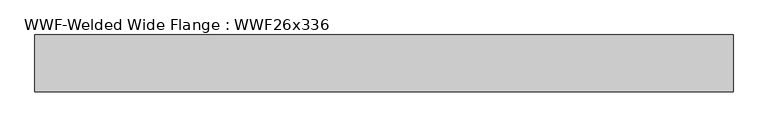
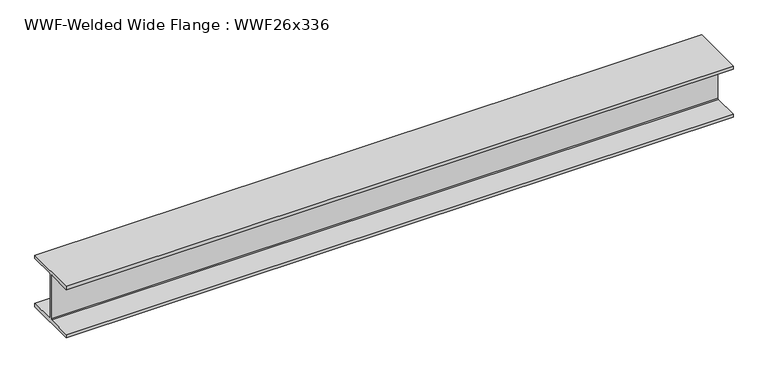
"""IFC4 building model written with IfcOpenShell, lengths in millimetres: beam geometry, WWF-Welded Wide Flange : WWF26x336."""

from ifc_helpers import new_model, si_unit, frame, origin, place, context, project, spatial, polyline, outline, extrude, source, transform, mapped, element, save


def wwf_welded_wide_flange_wwf26x336_095dbc8f(model_context):
    return source(origin(), model_context, "Body", "SweptSolid", [
        extrude(outline(polyline([(324.993, -284.988), (324.993, -324.993), (-324.993, -324.993), (-324.993, -284.988), (-20.6375, -284.988), (-9.9949, -274.3454), (-9.9949, 274.3454), (-20.6375, 284.988), (-324.993, 284.988), (-324.993, 324.993), (324.993, 324.993), (324.993, 284.988), (20.6375, 284.988), (9.9949, 274.3454), (9.9949, -274.3454), (20.6375, -284.988), (324.993, -284.988)])), frame((-3827.7582557, 0.0, 0.0), z_axis=(1.0, 0.0, 0.0), x_axis=(0.0, 1.0, 0.0)), (0.0, 0.0, 1.0), 7985.2423332),
    ])


if __name__ == "__main__":
    model = new_model("IFC4")
    model_context = context("Model", 3, world=origin())
    ifc_project = project(units=[si_unit("LENGTHUNIT", "METRE", prefix="MILLI")], contexts=[model_context])
    site = spatial("IfcSite", under=ifc_project)
    building = spatial("IfcBuilding", under=site)
    placement = place(None, origin())
    wwf_welded_wide_flange_wwf26x336_shape = wwf_welded_wide_flange_wwf26x336_095dbc8f(model_context)
    element("IfcBeam", 1, ObjectType="WWF-Welded Wide Flange : WWF26x336", at=placement, inside=building, context=model_context, shape_type="MappedRepresentation", body=[
        mapped(wwf_welded_wide_flange_wwf26x336_shape, transform((0.0, 0.0, 0.0), x_axis=(1.0, 0.0, 0.0), y_axis=(0.0, 1.0, 0.0), z_axis=(0.0, 0.0, 1.0))),
    ])
    save(model, "model.ifc")

# Revit data of these elements
# Type "WWF-Welded Wide Flange : WWF26x336"
#   Assembly Code = "B10"
#   Nominal d = "12"
#   W = 336
#   Length [instance default] = 1524 mm
#   bf = 649.986 mm
#   d = 649.986 mm
#   k = 20.638 mm
#   tf = 40.005 mm
#   tw = 19.99 mm
#   A = 0.0635483 m²
#   Structural Material [instance default] = Steel ASTM A572
# Element 1 (IfcBeam, "WWF-Welded Wide Flange : WWF26x336")
#   Structural Material = Metal - Steel 43-275
#   Materials on its faces: "Metal - Steel 43-275"
# Materials
#   "Steel ASTM A572": class "Metal", colour RGB 247 247 247, transparency 0, Description = "Structural steel, high strength low alloy, ASTM - A572 - 50", Cost = 0
#   "Metal - Steel 43-275": class "Metal", colour RGB 247 247 247, transparency 0, Cost = 0
